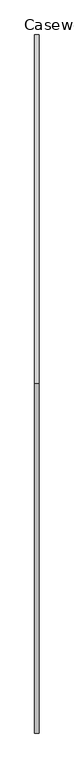
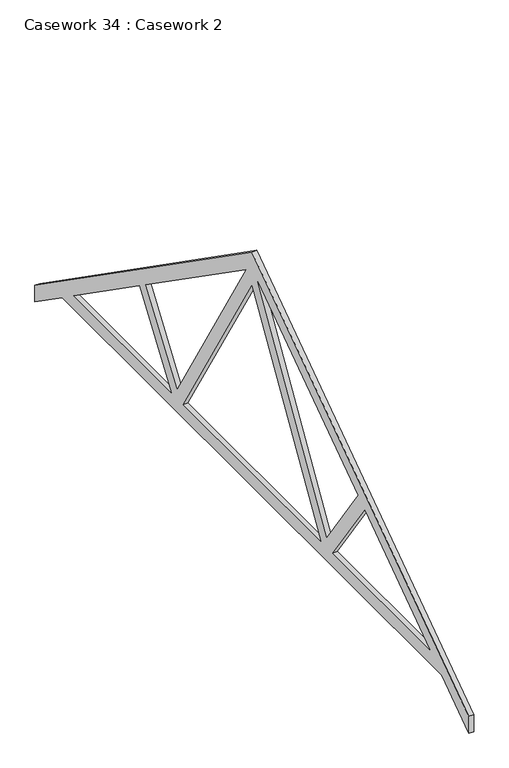
"""IFC4 building model written with IfcOpenShell, lengths in millimetres: furniture geometry, Casework 34 : Casework 2."""

import ifcopenshell
import ifcopenshell.guid

model = None  # the IFC model being written
_history = None  # IfcOwnerHistory: only IFC2X3 demands one
_inside = {}  # id of a spatial element -> (the spatial element, [elements in it])
_under = {}  # id of a project, library or spatial element -> (it, [spatial elements below it])
_declared = {}  # id of a project -> (the project, [libraries it declares])
_typed = {}  # id of a type object -> (the type object, [elements of that type])
_made_of = {}  # id of a material, layer set ... -> (it, [elements and type objects made of it])


def new_model(schema):
    """Start an empty IFC model of exactly this schema.

    Asked for "IFC4X3", IfcOpenShell would pick the latest addendum, in which some entities
    have other attributes; the version numbers below select the first issue.
    IFC2X3 requires an IfcOwnerHistory on every rooted entity: one is made here for all.
    """
    global model, _history
    if schema == "IFC4X3":
        model = ifcopenshell.file(schema_version=(4, 3, 0, 0))
    else:
        model = ifcopenshell.file(schema=schema)
    _inside.clear()
    _under.clear()
    _declared.clear()
    _typed.clear()
    _made_of.clear()
    _history = None
    if model.schema == "IFC2X3":
        org = make("IfcOrganization", Name="unknown")
        user = make(
            "IfcPersonAndOrganization",
            ThePerson=make("IfcPerson", FamilyName="unknown"),
            TheOrganization=org,
        )
        app = make(
            "IfcApplication",
            ApplicationDeveloper=org,
            Version="unknown",
            ApplicationFullName="unknown",
            ApplicationIdentifier="unknown",
        )
        _history = make(
            "IfcOwnerHistory",
            OwningUser=user,
            OwningApplication=app,
            ChangeAction="ADDED",
            CreationDate=0,
        )
    return model


def make(cls, **values):
    """One entity of the class cls with the attributes given. An attribute that is None is left unset."""
    return model.create_entity(
        cls, **{name: value for name, value in values.items() if value is not None}
    )


def rooted(cls, **values):
    """An entity with a GlobalId (a new one), such as an element, a storey or a relation."""
    return make(cls, GlobalId=ifcopenshell.guid.new(), OwnerHistory=_history, **values)


def si_unit(unit_type, name, prefix=None):
    """IfcSIUnit, for example si_unit("LENGTHUNIT", "METRE", prefix="MILLI")."""
    return make("IfcSIUnit", UnitType=unit_type, Prefix=prefix, Name=name)


def assignment(units):
    """IfcUnitAssignment: the units of a project."""
    return None if units is None else make("IfcUnitAssignment", Units=units)


def point(xyz):
    """IfcCartesianPoint."""
    return None if xyz is None else make("IfcCartesianPoint", Coordinates=xyz)


def direction(xyz):
    """IfcDirection."""
    return None if xyz is None else make("IfcDirection", DirectionRatios=xyz)


def frame(location, z_axis=None, x_axis=None):
    """IfcAxis2Placement3D, a coordinate frame: its origin and axes. An axis left out is left unset."""
    return make(
        "IfcAxis2Placement3D",
        Location=point(location),
        Axis=direction(z_axis),
        RefDirection=direction(x_axis),
    )


def origin():
    """The frame at (0, 0, 0) with its axes left unset."""
    return frame((0.0, 0.0, 0.0))


def place(relative_to, where):
    """IfcLocalPlacement: puts the frame where relative to a parent placement (None: the world)."""
    return make(
        "IfcLocalPlacement", PlacementRelTo=relative_to, RelativePlacement=where
    )


def context(
    kind, dimensions, precision=None, world=None, true_north=None, identifier=None
):
    """IfcGeometricRepresentationContext, for example the 3D "Model" context."""
    return make(
        "IfcGeometricRepresentationContext",
        ContextIdentifier=identifier,
        ContextType=kind,
        CoordinateSpaceDimension=dimensions,
        Precision=precision,
        WorldCoordinateSystem=world,
        TrueNorth=true_north,
    )


def project(units=None, contexts=None):
    """IfcProject with its units and contexts."""
    return rooted(
        "IfcProject",
        Name="project",
        RepresentationContexts=contexts,
        UnitsInContext=assignment(units),
    )


def spatial(cls, under=None, at=None, **own):
    """A site, building, storey or space (cls), placed at a placement, below another one or the project."""
    s = rooted(cls, ObjectPlacement=at, **own)
    if under is not None:
        _under.setdefault(under.id(), (under, []))[1].append(s)
    return s


def polyline(points):
    """IfcPolyline through the points."""
    return make("IfcPolyline", Points=[point(p) for p in points])


def outline(outer, holes=None, kind="AREA"):
    """IfcArbitraryClosedProfileDef: a profile drawn as a closed curve; with holes, ...WithVoids."""
    if holes is None:
        return make("IfcArbitraryClosedProfileDef", ProfileType=kind, OuterCurve=outer)
    return make(
        "IfcArbitraryProfileDefWithVoids",
        ProfileType=kind,
        OuterCurve=outer,
        InnerCurves=holes,
    )


def extrude(swept, where, along, depth):
    """IfcExtrudedAreaSolid: the profile swept, set in the frame where, extruded along a direction by depth."""
    return make(
        "IfcExtrudedAreaSolid",
        SweptArea=swept,
        Position=where,
        ExtrudedDirection=direction(along),
        Depth=depth,
    )


def shape(context_of_items, identifier, shape_type, items):
    """IfcShapeRepresentation: the items that make up one representation, for example the "Body"."""
    return make(
        "IfcShapeRepresentation",
        ContextOfItems=context_of_items,
        RepresentationIdentifier=identifier,
        RepresentationType=shape_type,
        Items=items,
    )


def source(mapping_origin, context_of_items, identifier, shape_type, items):
    """IfcRepresentationMap: a shape defined once, which mapped items show again and again."""
    return make(
        "IfcRepresentationMap",
        MappingOrigin=mapping_origin,
        MappedRepresentation=shape(context_of_items, identifier, shape_type, items),
    )


def transform(
    local_origin,
    x_axis=None,
    y_axis=None,
    z_axis=None,
    scale=None,
    scale2=None,
    scale3=None,
    uniform=True,
):
    """IfcCartesianTransformationOperator3D, or its non-uniform kind. x_axis, y_axis, z_axis: its Axis1, 2, 3."""
    if uniform:
        return make(
            "IfcCartesianTransformationOperator3D",
            Axis1=direction(x_axis),
            Axis2=direction(y_axis),
            LocalOrigin=point(local_origin),
            Scale=scale,
            Axis3=direction(z_axis),
        )
    return make(
        "IfcCartesianTransformationOperator3DnonUniform",
        Axis1=direction(x_axis),
        Axis2=direction(y_axis),
        LocalOrigin=point(local_origin),
        Scale=scale,
        Axis3=direction(z_axis),
        Scale2=scale2,
        Scale3=scale3,
    )


def mapped(mapping_source, mapping_target):
    """IfcMappedItem: shows the shape of a source again, moved by a transform."""
    return make(
        "IfcMappedItem", MappingSource=mapping_source, MappingTarget=mapping_target
    )


def made_of(thing, what):
    """Note that an element or type object is made of a material, layer set ...; save() writes the relation."""
    if what is not None:
        _made_of.setdefault(what.id(), (what, []))[1].append(thing)
    return thing


def element(
    cls,
    number,
    at=None,
    inside=None,
    cuts=None,
    type_object=None,
    material=None,
    context=None,
    identifier="Body",
    shape_type=None,
    held_by="IfcProductDefinitionShape",
    body=None,
    shapes=None,
    **own,
):
    """One element of the class cls, such as IfcWall. Its Tag is "e" and its number.

    at: its placement. inside: the storey or other place that contains it. cuts: it is an
    opening in that element (IfcRelVoidsElement). A single representation is given by context,
    identifier, shape_type and body (its items); several are given by shapes. held_by: the class
    of the entity that holds the representations. save() writes the other relations.
    """
    e = rooted(cls, Tag="e%d" % number, ObjectPlacement=at, **own)
    if body is not None:
        shapes = [shape(context, identifier, shape_type, body)]
    if shapes is not None:
        e.Representation = make(held_by, Representations=shapes)
    if inside is not None:
        _inside.setdefault(inside.id(), (inside, []))[1].append(e)
    if cuts is not None:
        rooted(
            "IfcRelVoidsElement", RelatingBuildingElement=cuts, RelatedOpeningElement=e
        )
    if type_object is not None:
        _typed.setdefault(type_object.id(), (type_object, []))[1].append(e)
    return made_of(e, material)


def aggregate(whole, parts):
    """IfcRelAggregates: a whole, such as a stair, and the parts it consists of."""
    return rooted("IfcRelAggregates", RelatingObject=whole, RelatedObjects=parts)


def save(model, path):
    """Write the relations noted so far, then the file.

    IfcRelAggregates (storeys below a building ...), IfcRelContainedInSpatialStructure (elements
    in a storey), IfcRelDefinesByType, IfcRelAssociatesMaterial and IfcRelDeclares: one each for
    every whole, place, type object, material and project.
    """
    for whole, parts in _under.values():
        aggregate(whole, parts)
    for where, things in _inside.values():
        rooted(
            "IfcRelContainedInSpatialStructure",
            RelatedElements=things,
            RelatingStructure=where,
        )
    for kind, things in _typed.values():
        rooted("IfcRelDefinesByType", RelatedObjects=things, RelatingType=kind)
    for what, things in _made_of.values():
        rooted("IfcRelAssociatesMaterial", RelatedObjects=things, RelatingMaterial=what)
    for by, libraries in _declared.values():
        rooted("IfcRelDeclares", RelatingContext=by, RelatedDefinitions=libraries)
    model.write(path)


def casework_34_casework_2_77ddbc4c(model_context):
    return source(origin(), model_context, "Body", "SweptSolid", [
        extrude(outline(polyline([(6583.1149316, 5285.0), (-277.3850684, 5285.0), (-767.3850684, 4941.8983063), (-767.3850684, 5125.0144946), (3152.8649316, 7870.0030963), (7073.1149316, 5125.0144946), (7073.1149316, 4941.8983063), (6583.1149316, 5285.0)]), holes=[polyline([(4612.3149663, 5435.0), (6368.8927306, 5435.0), (5190.2113591, 6260.3215815), (4612.3149663, 5435.0)]), polyline([(4394.2037684, 5435.0), (3152.8649316, 7500.9347567), (1911.5260948, 5435.0), (4394.2037684, 5435.0)]), polyline([(4504.5438357, 5542.6038939), (5067.3385525, 6346.3580469), (3262.0771677, 7610.415677), (4504.5438357, 5542.6038939)]), polyline([(1693.4148969, 5435.0), (1115.5185041, 6260.3215815), (-63.1628674, 5435.0), (1693.4148969, 5435.0)]), polyline([(1801.1860276, 5542.6038939), (3043.6526956, 7610.415677), (1238.3913108, 6346.3580469), (1801.1860276, 5542.6038939)])]), frame((-4421.5247381, 0.0, 0.0), z_axis=(1.0, 0.0, 0.0), x_axis=(0.0, 1.0, 0.0)), (0.0, 0.0, 1.0), 49.6351915),
    ])


if __name__ == "__main__":
    model = new_model("IFC4")
    model_context = context("Model", 3, world=origin())
    ifc_project = project(units=[si_unit("LENGTHUNIT", "METRE", prefix="MILLI")], contexts=[model_context])
    site = spatial("IfcSite", under=ifc_project)
    building = spatial("IfcBuilding", under=site)
    placement = place(None, origin())
    casework_34_casework_2_shape = casework_34_casework_2_77ddbc4c(model_context)
    element("IfcFurniture", 1, ObjectType="Casework 34 : Casework 2", at=placement, inside=building, context=model_context, shape_type="MappedRepresentation", body=[
        mapped(casework_34_casework_2_shape, transform((0.0, 0.0, 0.0), x_axis=(1.0, 0.0, 0.0), y_axis=(0.0, 1.0, 0.0), z_axis=(0.0, 0.0, 1.0))),
    ])
    save(model, "model.ifc")
